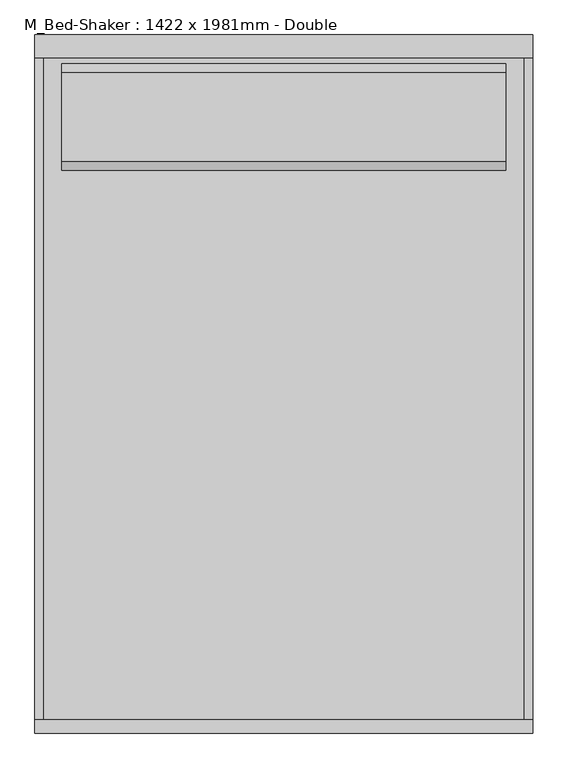
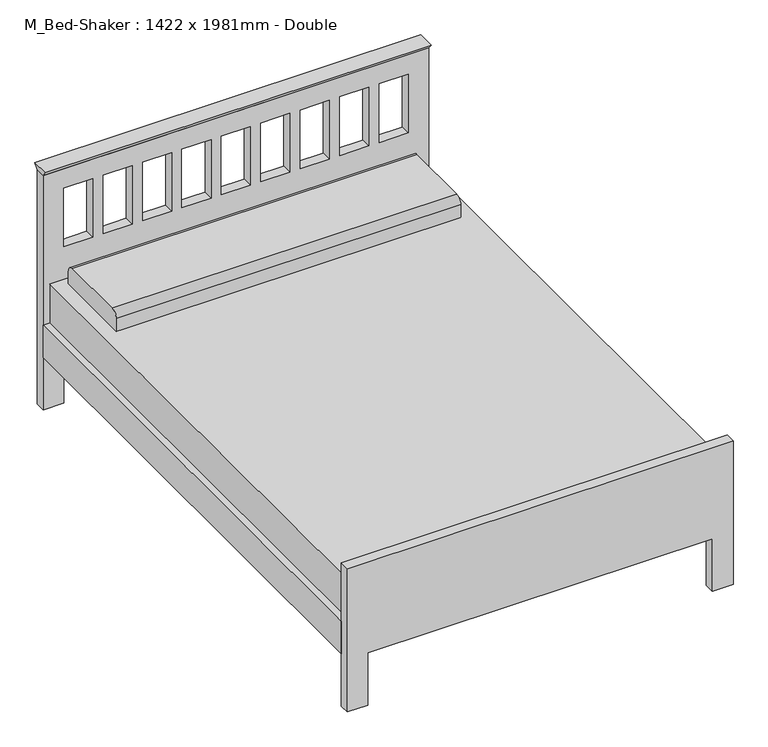
"""IFC4 building model written with IfcOpenShell, lengths in millimetres: furniture geometry, M_Bed-Shaker : 1422 x 1981mm - Double."""

from ifc_helpers import new_model, si_unit, point, frame, frame_2d, origin, place, context, project, spatial, polyline, circle_curve, trimmed, segment, composite_curve, outline, extrude, source, transform, mapped, element, save


def m_bed_shaker_1422_x_1981mm_double_096e7f55(model_context):
    return source(origin(), model_context, "Body", "SweptSolid", [
        extrude(outline(polyline([(-38.1, 914.4), (-51.9545455, 933.45), (13.8545455, 933.45), (0.0, 914.4), (-38.1, 914.4)])), frame((-730.0365546, 0.0, 0.0), z_axis=(1.0, 0.0, 0.0), x_axis=(0.0, 1.0, 0.0)), (0.0, 0.0, 1.0), 1422.4533613),
        extrude(outline(composite_curve([segment(polyline([(-373.2486637, 482.6), (-373.2486637, 533.4)]), True, "CONTINUOUS"), segment(trimmed(circle_curve(frame_2d((-347.8486637, 533.4)), 25.4), [point((-373.2486637, 533.4))], [point((-347.8486637, 558.8))], False, "CARTESIAN"), True, "CONTINUOUS"), segment(polyline([(-347.8486637, 558.8), (-93.8486637, 558.8)]), True, "CONTINUOUS"), segment(trimmed(circle_curve(frame_2d((-93.8486637, 533.4)), 25.4), [point((-93.8486637, 558.8))], [point((-68.4486637, 533.4))], False, "CARTESIAN"), True, "CONTINUOUS"), segment(polyline([(-68.4486637, 533.4), (-68.4486637, 482.6), (-373.2486637, 482.6)]), True, "CONTINUOUS")], self_intersect=False)), frame((-654.05, 0.0, 0.0), z_axis=(1.0, 0.0, 0.0), x_axis=(0.0, 1.0, 0.0)), (0.0, 0.0, 1.0), 1270.0),
        extrude(outline(polyline([(666.75, -38.1), (666.75, -1943.1), (-704.85, -1943.1), (-704.85, -38.1), (666.75, -38.1)])), frame((0.0, 0.0, 228.6), z_axis=(0.0, 0.0, 1.0), x_axis=(1.0, 0.0, 0.0)), (0.0, 0.0, 1.0), 254.0),
        extrude(outline(polyline([(666.75, -1943.1), (666.75, -38.1), (692.15, -38.1), (692.15, -1943.1), (666.75, -1943.1)])), frame((0.0, 0.0, 203.0994861), z_axis=(0.0, 0.0, 1.0), x_axis=(1.0, 0.0, 0.0)), (0.0, 0.0, 1.0), 127.0),
        extrude(outline(polyline([(-730.25, -1943.1), (-730.25, -38.1), (-704.85, -38.1), (-704.85, -1943.1), (-730.25, -1943.1)])), frame((0.0, 0.0, 203.5755296), z_axis=(0.0, 0.0, 1.0), x_axis=(1.0, 0.0, 0.0)), (0.0, 0.0, 1.0), 127.0),
        extrude(outline(polyline([(0.0, -654.05), (203.2, -654.05), (203.2, 615.95), (0.0, 615.95), (0.0, 692.15), (558.8, 692.15), (558.8, -730.25), (0.0, -730.25), (0.0, -654.05)])), frame((0.0, -1981.2, 0.0), z_axis=(0.0, 1.0, 0.0), x_axis=(0.0, 0.0, 1.0)), (0.0, 0.0, 1.0), 38.1),
        extrude(outline(polyline([(914.4, 692.4168067), (914.4, -730.0365546), (0.0, -730.0365546), (0.0, -654.05), (203.2, -654.05), (203.2, 615.95), (0.0, 615.95), (0.0, 692.4168067), (914.4, 692.4168067)]), holes=[polyline([(838.2, -546.8055556), (609.6, -546.8055556), (609.6, -654.05), (838.2, -654.05), (838.2, -546.8055556)]), polyline([(838.2, -401.4611111), (609.6, -401.4611111), (609.6, -508.7055556), (838.2, -508.7055556), (838.2, -401.4611111)]), polyline([(838.2, -256.1166667), (609.6, -256.1166667), (609.6, -363.3611111), (838.2, -363.3611111), (838.2, -256.1166667)]), polyline([(838.2, -110.7722222), (609.6, -110.7722222), (609.6, -218.0166667), (838.2, -218.0166667), (838.2, -110.7722222)]), polyline([(838.2, 179.9166667), (609.6, 179.9166667), (609.6, 72.6722222), (838.2, 72.6722222), (838.2, 179.9166667)]), polyline([(838.2, 325.2611111), (609.6, 325.2611111), (609.6, 218.0166667), (838.2, 218.0166667), (838.2, 325.2611111)]), polyline([(838.2, 470.6055556), (609.6, 470.6055556), (609.6, 363.3611111), (838.2, 363.3611111), (838.2, 470.6055556)]), polyline([(838.2, 615.95), (609.6, 615.95), (609.6, 508.7055556), (838.2, 508.7055556), (838.2, 615.95)]), polyline([(838.2, 34.5722222), (609.6, 34.5722222), (609.6, -72.6722222), (838.2, -72.6722222), (838.2, 34.5722222)])]), frame((0.0, -38.1, 0.0), z_axis=(0.0, 1.0, 0.0), x_axis=(0.0, 0.0, 1.0)), (0.0, 0.0, 1.0), 38.1),
    ])


if __name__ == "__main__":
    model = new_model("IFC4")
    model_context = context("Model", 3, world=origin())
    ifc_project = project(units=[si_unit("LENGTHUNIT", "METRE", prefix="MILLI")], contexts=[model_context])
    site = spatial("IfcSite", under=ifc_project)
    building = spatial("IfcBuilding", under=site)
    placement = place(None, origin())
    m_bed_shaker_1422_x_1981mm_double_shape = m_bed_shaker_1422_x_1981mm_double_096e7f55(model_context)
    element("IfcFurniture", 1, ObjectType="M_Bed-Shaker : 1422 x 1981mm - Double", at=placement, inside=building, context=model_context, shape_type="MappedRepresentation", body=[
        mapped(m_bed_shaker_1422_x_1981mm_double_shape, transform((0.0, 0.0, 0.0), x_axis=(1.0, 0.0, 0.0), y_axis=(0.0, 1.0, 0.0), z_axis=(0.0, 0.0, 1.0))),
    ])
    save(model, "model.ifc")

# Revit data of these elements
# Type "M_Bed-Shaker : 1422 x 1981mm - Double"
#   Length = 1.9812 m
#   Width = 1.4224 m
#   Frame Material = Birch
#   Mattress Material = Linen, White
# Element 1 (IfcFurniture, "M_Bed-Shaker : 1422 x 1981mm - Double")
#   Materials on its faces: "Birch", "Linen, White"
# Materials
#   "Birch": class "Wood", colour RGB 224 178 126, transparency 0, Description = "Betula Alleghaniensis", Cost = 0
#   "Linen, White": class "Textile", colour RGB 247 247 239, transparency 0, Description = "Linen, white", Cost = 0
